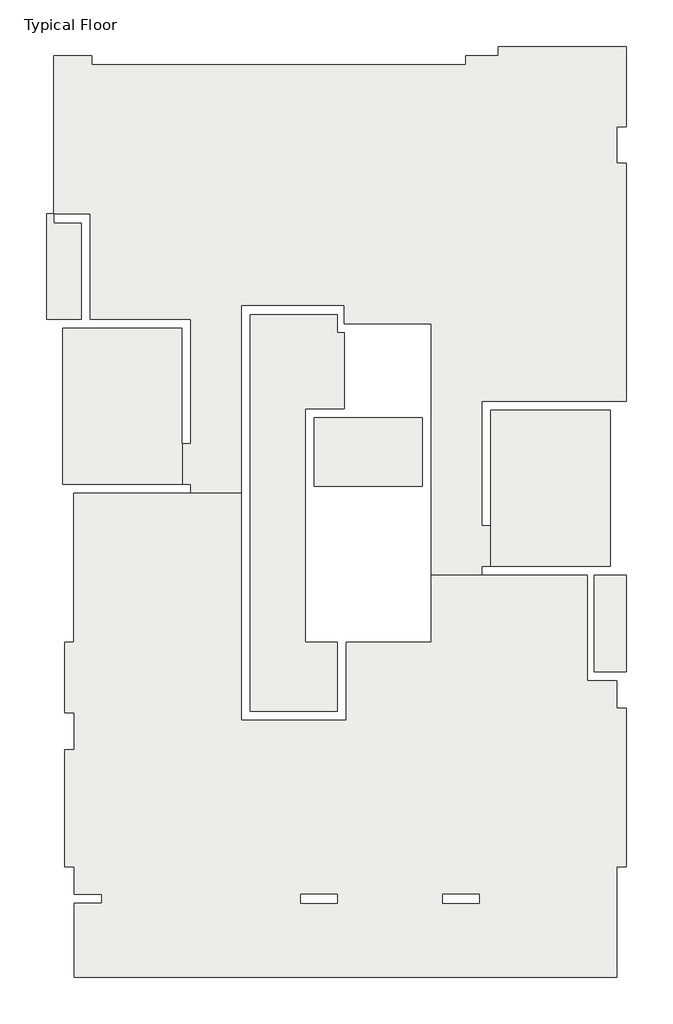
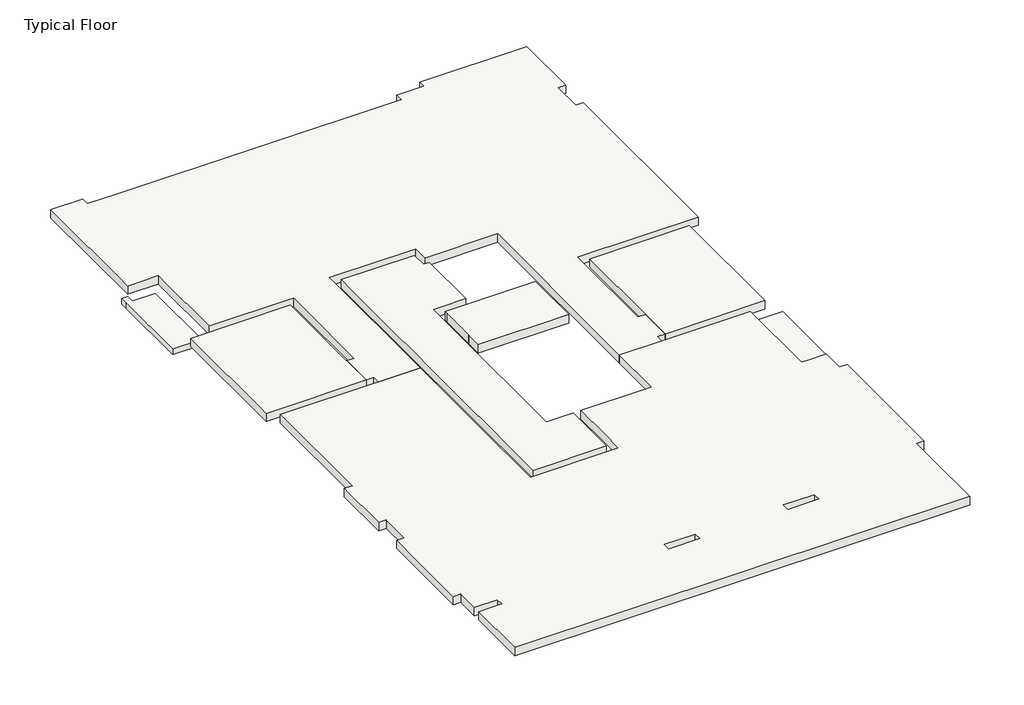
# One storey: 8 slabs.
"""IFC4 building model written with IfcOpenShell, lengths in millimetres."""

from ifc_helpers import new_model, si_unit, frame, origin, place, context, project, spatial, polyline, outline, extrude, faceted_brep, element, save

model = new_model("IFC4")

# Units and contexts
model_context = context("Model", 3, world=origin())
ifc_project = project(units=[si_unit("LENGTHUNIT", "METRE", prefix="MILLI")], contexts=[model_context])

# Site, building, storey
site = spatial("IfcSite", under=ifc_project)
building = spatial("IfcBuilding", under=site)
storey = spatial("IfcBuildingStorey", under=building, Name="Typical Floor", Elevation=3150.0)

# Slabs
placement = place(None, origin())
element("IfcSlab", 1, ObjectType="15", at=placement, inside=storey, context=model_context, shape_type="SweptSolid", body=[
    extrude(outline(polyline([(-8245.045869, 24273.2318976), (-8245.045869, 22171.4624057), (-8943.1419846, 22171.4624057), (-8943.1419846, 24273.2318976), (-8245.045869, 24273.2318976)])), frame((0.0, 0.0, 2700.0), z_axis=(0.0, 0.0, 1.0), x_axis=(1.0, 0.0, 0.0)), (0.0, 0.0, 1.0), 150.0),
])
element("IfcSlab", 2, ObjectType="15", at=placement, inside=storey, context=model_context, shape_type="SweptSolid", body=[
    extrude(outline(polyline([(-20134.1305711, 31959.1185492), (-20134.1305711, 29864.251036), (-20886.1283922, 29864.251036), (-20886.1283922, 31959.1185492), (-20886.1283922, 32159.1185492), (-20734.1305711, 32159.1185492), (-20734.1305711, 31959.1185492), (-20134.1305711, 31959.1185492)])), frame((0.0, 0.0, 2700.0), z_axis=(0.0, 0.0, 1.0), x_axis=(1.0, 0.0, 0.0)), (0.0, 0.0, 1.0), 150.0),
])
element("IfcSlab", 3, ObjectType="23", at=placement, inside=storey, context=model_context, shape_type="Brep", body=[
    faceted_brep([(-8593.0697613, 27874.251036, 2920.0), (-8593.0697613, 24473.2318976, 2920.0), (-11192.3056926, 24473.2318976, 2920.0), (-11192.3056926, 25350.9157719, 2920.0), (-11192.3056926, 27874.251036, 2920.0), (-8593.0697613, 27874.251036, 3150.0), (-11192.3056926, 27874.251036, 3150.0), (-11192.3056926, 25350.9157719, 3150.0), (-11192.3056926, 24473.2318976, 3150.0), (-8593.0697613, 24473.2318976, 3150.0)], [[[0, 1, 2, 3, 4]], [[5, 6, 7, 8, 9]], [[1, 0, 5, 9]], [[2, 1, 9, 8]], [[4, 3, 2, 8, 7, 6]], [[0, 4, 6, 5]]]),
])
element("IfcSlab", 4, ObjectType="23", at=placement, inside=storey, context=model_context, shape_type="SweptSolid", body=[
    extrude(outline(polyline([(-17926.892461, 26263.2318976), (-20536.1283922, 26263.2318976), (-20536.1283922, 29664.251036), (-17936.892461, 29664.251036), (-17936.892461, 27140.9157719), (-17926.892461, 27140.9157719), (-17926.892461, 26263.2318976)])), frame((0.0, 0.0, 2920.0), z_axis=(0.0, 0.0, 1.0), x_axis=(1.0, 0.0, 0.0)), (0.0, 0.0, 1.0), 230.0),
])
element("IfcSlab", 5, ObjectType="23", at=placement, inside=storey, context=model_context, shape_type="Brep", body=[
    faceted_brep([(-15241.6888164, 22813.9119334, 2920.0), (-14543.2190847, 22813.9119334, 2920.0), (-14543.2190847, 21764.1541281, 2920.0), (-14543.2190847, 21314.7324543, 2920.0), (-16442.902761, 21314.7324543, 2920.0), (-16442.902761, 29962.1790859, 2920.0), (-14542.0990768, 29962.1790859, 2920.0), (-14542.0990768, 29561.6748888, 2920.0), (-14392.0990768, 29561.6748888, 2920.0), (-14392.0990768, 27911.3754017, 2920.0), (-15041.6888164, 27911.3754017, 2920.0), (-15241.6888164, 27911.3754017, 2920.0), (-15241.6888164, 27611.1233031, 2920.0), (-15241.6888164, 26638.171559, 2920.0), (-15241.6888164, 23013.9119334, 2920.0), (-14543.2190847, 22813.9119334, 3150.0), (-15241.6888164, 22813.9119334, 3150.0), (-15241.6888164, 23013.9119334, 3150.0), (-15241.6888164, 26638.171559, 3150.0), (-15241.6888164, 27611.1233031, 3150.0), (-15241.6888164, 27911.3754017, 3150.0), (-15041.6888164, 27911.3754017, 3150.0), (-14392.0990768, 27911.3754017, 3150.0), (-14392.0990768, 29561.6748888, 3150.0), (-14542.0990768, 29561.6748888, 3150.0), (-14542.0990768, 29962.1790859, 3150.0), (-16442.902761, 29962.1790859, 3150.0), (-16442.902761, 24264.0058702, 3150.0), (-16442.902761, 23263.128057, 3150.0), (-16442.902761, 21314.7324543, 3150.0), (-14543.2190847, 21314.7324543, 3150.0), (-14543.2190847, 21764.1541281, 3150.0)], [[[0, 1, 2, 3, 4, 5, 6, 7, 8, 9, 10, 11, 12, 13, 14]], [[15, 16, 17, 18, 19, 20, 21, 22, 23, 24, 25, 26, 27, 28, 29, 30, 31]], [[20, 11, 10, 9, 22, 21]], [[11, 20, 19, 18, 17, 16, 0, 14, 13, 12]], [[1, 0, 16, 15]], [[1, 15, 31, 30, 3, 2]], [[4, 3, 30, 29]], [[5, 4, 29, 28, 27, 26]], [[6, 5, 26, 25]], [[7, 6, 25, 24]], [[8, 7, 24, 23]], [[9, 8, 23, 22]]]),
])
element("IfcSlab", 6, ObjectType="23", at=placement, inside=storey, context=model_context, shape_type="SweptSolid", body=[
    extrude(outline(polyline([(-12692.7515319, 27711.3754017), (-12692.7515319, 26212.2334071), (-15041.6888164, 26212.2334071), (-15041.6888164, 26638.171559), (-15046.6888164, 26638.171559), (-15046.6888164, 27611.1233031), (-15041.6888164, 27611.1233031), (-15041.6888164, 27711.3754017), (-12692.7515319, 27711.3754017)])), frame((0.0, 0.0, 2920.0), z_axis=(0.0, 0.0, 1.0), x_axis=(1.0, 0.0, 0.0)), (0.0, 0.0, 1.0), 230.0),
])
element("IfcSlab", 7, ObjectType="23", at=placement, inside=storey, context=model_context, shape_type="Brep", body=[
    faceted_brep([(-8245.045869, 35808.9801951, 2920.0), (-8245.045869, 34060.248461, 2920.0), (-8445.045869, 34060.248461, 2920.0), (-8445.045869, 33260.248461, 2920.0), (-8245.045869, 33260.248461, 2920.0), (-8245.045869, 28074.251036, 2920.0), (-11392.3056926, 28074.251036, 2920.0), (-11392.3056926, 27874.251036, 2920.0), (-11392.3056926, 25350.9157719, 2920.0), (-11192.3056926, 25350.9157719, 2920.0), (-11192.3056926, 24473.2318976, 2920.0), (-11392.3056926, 24473.2318976, 2920.0), (-11392.3056926, 24273.2318976, 2920.0), (-12492.7515319, 24273.2318976, 2920.0), (-12492.7515319, 29561.6748888, 2920.0), (-12492.7515319, 29761.6748888, 2920.0), (-14392.0990768, 29761.6748888, 2920.0), (-14392.0990768, 30162.1790859, 2920.0), (-14542.0990768, 30162.1790859, 2920.0), (-16442.902761, 30162.1790859, 2920.0), (-16642.902761, 30162.1790859, 2920.0), (-16642.902761, 26063.2318976, 2920.0), (-17736.892461, 26063.2318976, 2920.0), (-17736.892461, 26263.2318976, 2920.0), (-17926.892461, 26263.2318976, 2920.0), (-17926.892461, 27140.9157719, 2920.0), (-17736.892461, 27140.9157719, 2920.0), (-17736.892461, 29664.251036, 2920.0), (-17736.892461, 29864.251036, 2920.0), (-19934.1305711, 29864.251036, 2920.0), (-19934.1305711, 31959.1185492, 2920.0), (-19934.1305711, 32159.1185492, 2920.0), (-20734.1305711, 32159.1185492, 2920.0), (-20734.1305711, 35608.8121294, 2920.0), (-19901.5564046, 35608.8121294, 2920.0), (-19901.5564046, 35408.8121294, 2920.0), (-19101.5564046, 35408.8121294, 2920.0), (-11741.5564046, 35408.8121294, 2920.0), (-11741.5564046, 35608.9801951, 2920.0), (-11033.3239157, 35608.9801951, 2920.0), (-11033.3239157, 35808.9801951, 2920.0), (-8245.045869, 34060.248461, 3150.0), (-8245.045869, 35808.9801951, 3150.0), (-11033.3239157, 35808.9801951, 3150.0), (-11033.3239157, 35608.9801951, 3150.0), (-11741.5564046, 35608.9801951, 3150.0), (-11741.5564046, 35608.8121294, 3150.0), (-11741.5564046, 35408.8121294, 3150.0), (-19101.5564046, 35408.8121294, 3150.0), (-19901.5564046, 35408.8121294, 3150.0), (-19901.5564046, 35608.8121294, 3150.0), (-20734.1305711, 35608.8121294, 3150.0), (-20734.1305711, 32159.1185492, 3150.0), (-19934.1305711, 32159.1185492, 3150.0), (-19934.1305711, 31959.1185492, 3150.0), (-19934.1305711, 29864.251036, 3150.0), (-17736.892461, 29864.251036, 3150.0), (-17736.892461, 29664.251036, 3150.0), (-17736.892461, 27140.9157719, 3150.0), (-17926.892461, 27140.9157719, 3150.0), (-17926.892461, 26263.2318976, 3150.0), (-17736.892461, 26263.2318976, 3150.0), (-17736.892461, 26063.2318976, 3150.0), (-16642.902761, 26063.2318976, 3150.0), (-16642.902761, 30162.1790859, 3150.0), (-16442.902761, 30162.1790859, 3150.0), (-14542.0990768, 30162.1790859, 3150.0), (-14392.0990768, 30162.1790859, 3150.0), (-14392.0990768, 29761.6748888, 3150.0), (-12492.7515319, 29761.6748888, 3150.0), (-12492.7515319, 29561.6748888, 3150.0), (-12492.7515319, 24273.2318976, 3150.0), (-11392.3056926, 24273.2318976, 3150.0), (-11392.3056926, 24473.2318976, 3150.0), (-11192.3056926, 24473.2318976, 3150.0), (-11192.3056926, 25350.9157719, 3150.0), (-11392.3056926, 25350.9157719, 3150.0), (-11392.3056926, 27874.251036, 3150.0), (-11392.3056926, 28074.251036, 3150.0), (-8245.045869, 28074.251036, 3150.0), (-8245.045869, 33260.248461, 3150.0), (-8445.045869, 33260.248461, 3150.0), (-8445.045869, 34060.248461, 3150.0)], [[[0, 1, 2, 3, 4, 5, 6, 7, 8, 9, 10, 11, 12, 13, 14, 15, 16, 17, 18, 19, 20, 21, 22, 23, 24, 25, 26, 27, 28, 29, 30, 31, 32, 33, 34, 35, 36, 37, 38, 39, 40]], [[41, 42, 43, 44, 45, 46, 47, 48, 49, 50, 51, 52, 53, 54, 55, 56, 57, 58, 59, 60, 61, 62, 63, 64, 65, 66, 67, 68, 69, 70, 71, 72, 73, 74, 75, 76, 77, 78, 79, 80, 81, 82]], [[1, 0, 42, 41]], [[2, 1, 41, 82]], [[3, 2, 82, 81]], [[4, 3, 81, 80]], [[5, 4, 80, 79]], [[6, 5, 79, 78]], [[6, 78, 77, 76, 8, 7]], [[9, 8, 76, 75]], [[10, 9, 75, 74]], [[11, 10, 74, 73]], [[12, 11, 73, 72]], [[13, 12, 72, 71]], [[13, 71, 70, 69, 15, 14]], [[16, 15, 69, 68]], [[17, 16, 68, 67]], [[17, 67, 66, 65, 64, 20, 19, 18]], [[21, 20, 64, 63]], [[22, 21, 63, 62]], [[23, 22, 62, 61]], [[23, 61, 60, 24]], [[58, 26, 25, 59]], [[26, 58, 57, 56, 28, 27]], [[29, 28, 56, 55]], [[29, 55, 54, 53, 31, 30]], [[32, 31, 53, 52]], [[33, 32, 52, 51]], [[34, 33, 51, 50]], [[35, 34, 50, 49]], [[35, 49, 48, 47, 37, 36]], [[37, 47, 46, 45, 38]], [[43, 40, 39, 44]], [[0, 40, 43, 42]], [[44, 39, 38, 45]], [[25, 24, 60, 59]]]),
])
element("IfcSlab", 8, ObjectType="23", at=placement, inside=storey, context=model_context, shape_type="Brep", body=[
    faceted_brep([(-12492.7515319, 22813.9119334, 2920.0), (-12492.7515319, 24273.2318976, 2920.0), (-11392.3056926, 24273.2318976, 2920.0), (-9093.1419846, 24273.2318976, 2920.0), (-9093.1419846, 21971.29434, 2920.0), (-8445.045869, 21971.29434, 2920.0), (-8445.045869, 21371.4624057, 2920.0), (-8245.045869, 21371.4624057, 2920.0), (-8245.045869, 17914.2549976, 2920.0), (-8445.045869, 17914.2549976, 2920.0), (-8445.045869, 17114.2549976, 2920.0), (-8445.045869, 15502.6614945, 2920.0), (-20285.7922608, 15502.6614945, 2920.0), (-20285.7922608, 17115.8692988, 2920.0), (-20285.7922608, 17116.0748491, 2920.0), (-19685.7922608, 17116.0748491, 2920.0), (-19685.7922608, 17316.0748491, 2920.0), (-20285.7922608, 17316.0748491, 2920.0), (-20285.7922608, 17914.2549976, 2920.0), (-20485.7922608, 17914.2549976, 2920.0), (-20485.7922608, 20472.3204112, 2920.0), (-20285.7922608, 20472.3204112, 2920.0), (-20285.7922608, 21272.3204112, 2920.0), (-20487.9482438, 21272.3204112, 2920.0), (-20487.9482438, 22813.9119334, 2920.0), (-20287.9482438, 22813.9119334, 2920.0), (-20287.9482438, 26063.2318976, 2920.0), (-17736.892461, 26063.2318976, 2920.0), (-16642.902761, 26063.2318976, 2920.0), (-16642.902761, 24264.0058702, 2920.0), (-16642.902761, 23263.128057, 2920.0), (-16642.902761, 21314.7324543, 2920.0), (-16642.902761, 21114.7324543, 2920.0), (-14543.2190847, 21114.7324543, 2920.0), (-14343.2190847, 21114.7324543, 2920.0), (-14343.2190847, 21764.1541281, 2920.0), (-14343.2190847, 22813.9119334, 2920.0), (-12692.7515319, 22813.9119334, 2920.0), (-11442.9937266, 17316.0748491, 2920.0), (-12242.9937266, 17316.0748491, 2920.0), (-12242.9937266, 17116.0748491, 2920.0), (-11442.9937266, 17116.0748491, 2920.0), (-14541.7353646, 17316.0748491, 2920.0), (-15341.7353646, 17316.0748491, 2920.0), (-15341.7353646, 17116.0748491, 2920.0), (-14541.7353646, 17116.0748491, 2920.0), (-12492.7515319, 24273.2318976, 3150.0), (-12492.7515319, 22813.9119334, 3150.0), (-12692.7515319, 22813.9119334, 3150.0), (-14343.2190847, 22813.9119334, 3150.0), (-14343.2190847, 21764.1541281, 3150.0), (-14343.2190847, 21114.7324543, 3150.0), (-14543.2190847, 21114.7324543, 3150.0), (-16642.902761, 21114.7324543, 3150.0), (-16642.902761, 21314.7324543, 3150.0), (-16642.902761, 23263.128057, 3150.0), (-16642.902761, 24264.0058702, 3150.0), (-16642.902761, 26063.2318976, 3150.0), (-17736.892461, 26063.2318976, 3150.0), (-20287.9482438, 26063.2318976, 3150.0), (-20287.9482438, 22813.9119334, 3150.0), (-20487.9482438, 22813.9119334, 3150.0), (-20487.9482438, 21272.3204112, 3150.0), (-20485.7922608, 21272.3204112, 3150.0), (-20285.7922608, 21272.3204112, 3150.0), (-20285.7922608, 20472.3204112, 3150.0), (-20485.7922608, 20472.3204112, 3150.0), (-20485.7922608, 17914.2549976, 3150.0), (-20285.7922608, 17914.2549976, 3150.0), (-20285.7922608, 17316.0748491, 3150.0), (-19685.7922608, 17316.0748491, 3150.0), (-19685.7922608, 17116.0748491, 3150.0), (-20285.7922608, 17116.0748491, 3150.0), (-20285.7922608, 17115.8692988, 3150.0), (-20285.7922608, 15502.6614945, 3150.0), (-8445.045869, 15502.6614945, 3150.0), (-8445.045869, 17114.2549976, 3150.0), (-8445.045869, 17914.2549976, 3150.0), (-8245.045869, 17914.2549976, 3150.0), (-8245.045869, 21371.4624057, 3150.0), (-8445.045869, 21371.4624057, 3150.0), (-8445.045869, 21971.29434, 3150.0), (-8943.1419846, 21971.29434, 3150.0), (-9093.1419846, 21971.29434, 3150.0), (-9093.1419846, 24273.2318976, 3150.0), (-11392.3056926, 24273.2318976, 3150.0), (-12242.9937266, 17316.0748491, 3150.0), (-11442.9937266, 17316.0748491, 3150.0), (-11442.9937266, 17116.0748491, 3150.0), (-12242.9937266, 17116.0748491, 3150.0), (-15341.7353646, 17316.0748491, 3150.0), (-14541.7353646, 17316.0748491, 3150.0), (-14541.7353646, 17116.0748491, 3150.0), (-15341.7353646, 17116.0748491, 3150.0)], [[[0, 1, 2, 3, 4, 5, 6, 7, 8, 9, 10, 11, 12, 13, 14, 15, 16, 17, 18, 19, 20, 21, 22, 23, 24, 25, 26, 27, 28, 29, 30, 31, 32, 33, 34, 35, 36, 37], [38, 39, 40, 41], [42, 43, 44, 45]], [[46, 47, 48, 49, 50, 51, 52, 53, 54, 55, 56, 57, 58, 59, 60, 61, 62, 63, 64, 65, 66, 67, 68, 69, 70, 71, 72, 73, 74, 75, 76, 77, 78, 79, 80, 81, 82, 83, 84, 85], [86, 87, 88, 89], [90, 91, 92, 93]], [[53, 32, 31, 30, 29, 28, 57, 56, 55, 54]], [[32, 53, 52, 51, 34, 33]], [[34, 51, 50, 49, 36, 35]], [[36, 49, 48, 47, 0, 37]], [[1, 0, 47, 46]], [[1, 46, 85, 84, 3, 2]], [[4, 3, 84, 83]], [[5, 4, 83, 82, 81]], [[6, 5, 81, 80]], [[7, 6, 80, 79]], [[8, 7, 79, 78]], [[9, 8, 78, 77]], [[9, 77, 76, 75, 11, 10]], [[12, 11, 75, 74]], [[12, 74, 73, 72, 14, 13]], [[70, 16, 15, 71]], [[17, 16, 70, 69]], [[18, 17, 69, 68]], [[19, 18, 68, 67]], [[20, 19, 67, 66]], [[20, 66, 65, 21]], [[62, 23, 22, 64, 63]], [[24, 23, 62, 61]], [[25, 24, 61, 60]], [[25, 60, 59, 26]], [[38, 87, 86, 39]], [[87, 38, 41, 88]], [[88, 41, 40, 89]], [[89, 40, 39, 86]], [[42, 91, 90, 43]], [[91, 42, 45, 92]], [[92, 45, 44, 93]], [[93, 44, 43, 90]], [[71, 15, 14, 72]], [[64, 22, 21, 65]], [[26, 59, 58, 57, 28, 27]]]),
])

save(model, "model.ifc")

# Revit data of these elements
# Type "15"
#   Function = 0
#   Layers, outside or top first: 15 cm "Concrete" (function 1)
# Type "23"
#   Function = 0
#   Layers, outside or top first: 23 cm "Concrete" (function 1)
# Element 1 (IfcSlab, "15")
#   Mark = "S1"
#   SOFiSTiK_AMG_Comments = ""
#   Height Offset From Level = -30 cm
#   built-in parameter 1001954 = 1
#   SOFiSTiK_AMG_Scheduled = yes
#   SOFiSTiK_AMG_Adjusted = yes
#   Phase Created = New Construction
#   Materials on its faces: "Concrete"
# Element 2 (IfcSlab, "15")
#   Mark = "S2"
#   SOFiSTiK_AMG_Comments = ""
#   built-in parameter 1001955 = 1.5708 (stored number, unit not read)
#   Height Offset From Level = -30 cm
#   built-in parameter 1001954 = 1
#   SOFiSTiK_AMG_Scheduled = yes
#   SOFiSTiK_AMG_Adjusted = yes
#   Phase Created = New Construction
#   Materials on its faces: "Concrete"
# Element 3 (IfcSlab, "23")
#   Mark = "S3"
#   SOFiSTiK_AMG_Comments = ""
#   Height Offset From Level = 0 cm
#   built-in parameter 1001954 = 1
#   SOFiSTiK_AMG_Scheduled = yes
#   SOFiSTiK_AMG_Adjusted = yes
#   Phase Created = New Construction
#   Materials on its faces: "Concrete"
# Element 4 (IfcSlab, "23")
#   Mark = "S4"
#   SOFiSTiK_AMG_Comments = ""
#   Height Offset From Level = 0 cm
#   built-in parameter 1001954 = 1
#   SOFiSTiK_AMG_Scheduled = yes
#   SOFiSTiK_AMG_Adjusted = yes
#   Phase Created = New Construction
#   Materials on its faces: "Concrete"
# Element 5 (IfcSlab, "23")
#   Mark = "S5"
#   SOFiSTiK_AMG_Comments = ""
#   built-in parameter 1001955 = -1.5708 (stored number, unit not read)
#   Height Offset From Level = 0 cm
#   built-in parameter 1001954 = 1
#   SOFiSTiK_AMG_Scheduled = yes
#   SOFiSTiK_AMG_Adjusted = yes
#   Phase Created = New Construction
#   Materials on its faces: "Concrete"
# Element 6 (IfcSlab, "23")
#   Mark = "S6"
#   SOFiSTiK_AMG_Comments = ""
#   Height Offset From Level = 0 cm
#   built-in parameter 1001954 = 1
#   SOFiSTiK_AMG_Scheduled = yes
#   SOFiSTiK_AMG_Adjusted = yes
#   Phase Created = New Construction
#   Materials on its faces: "Concrete"
# Element 7 (IfcSlab, "23")
#   Mark = "S7"
#   SOFiSTiK_AMG_Comments = ""
#   Height Offset From Level = 0 cm
#   built-in parameter 1001954 = 1
#   SOFiSTiK_AMG_Scheduled = yes
#   SOFiSTiK_AMG_Adjusted = yes
#   Phase Created = New Construction
#   Materials on its faces: "Concrete"
# Element 8 (IfcSlab, "23")
#   Mark = "S8"
#   SOFiSTiK_AMG_Comments = ""
#   Height Offset From Level = 0 cm
#   built-in parameter 1001954 = 1
#   SOFiSTiK_AMG_Scheduled = yes
#   SOFiSTiK_AMG_Adjusted = no
#   Phase Created = New Construction
#   Materials on its faces: "Concrete"
# Materials
#   "Concrete": class "Concrete", colour RGB 192 192 192, transparency 0, Keynote = "01000", Description = "Cast-in-place concrete", Cost = 0
